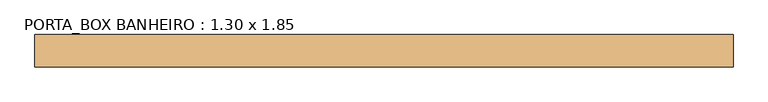
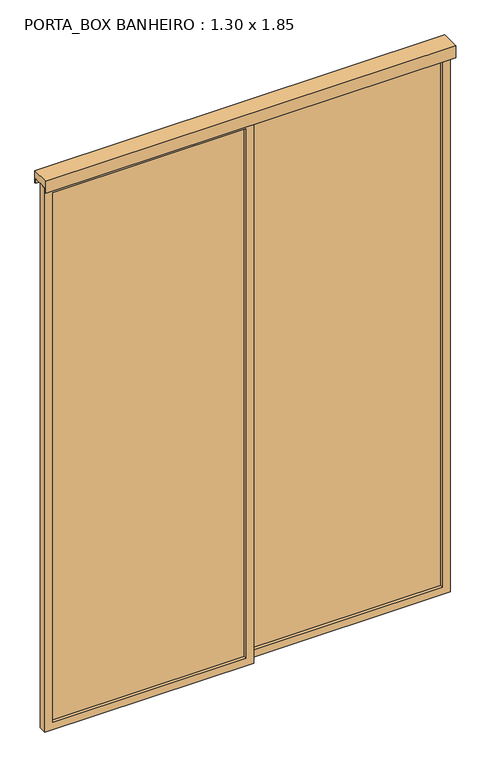
"""IFC4 building model written with IfcOpenShell, lengths in millimetres: door geometry, PORTA_BOX BANHEIRO : 1.30 x 1.85."""

from ifc_helpers import new_model, si_unit, frame, origin, place, context, project, spatial, polyline, outline, extrude, faceted_brep, source, transform, mapped, element, save


def porta_box_banheiro_1_30_x_1_85_4d29e14f(model_context):
    return source(origin(), model_context, "Body", "SolidModel", [
        extrude(outline(polyline([(652.5, 15.0), (652.5, 10.0), (10.0, 10.0), (10.0, 15.0), (652.5, 15.0)])), frame((0.0, 0.0, 10.0), z_axis=(0.0, 0.0, 1.0), x_axis=(1.0, 0.0, 0.0)), (0.0, 0.0, 1.0), 1805.0),
        faceted_brep([(637.5, 15.0, 1800.0), (637.5, 25.0, 1800.0), (637.5, 25.0, 25.0), (637.5, 15.0, 25.0), (662.5, 25.0, 1825.0), (662.5, 25.0, 0.0), (0.0, 25.0, 0.0), (0.0, 25.0, 1825.0), (25.0, 25.0, 1800.0), (25.0, 25.0, 25.0), (25.0, 15.0, 25.0), (10.0, 15.0, 1815.0), (10.0, 15.0, 10.0), (652.5, 15.0, 10.0), (652.5, 15.0, 1815.0), (25.0, 15.0, 1800.0), (662.5, 0.0, 1825.0), (662.5, 0.0, 0.0), (0.0, 0.0, 1825.0), (0.0, 0.0, 0.0), (637.5, 0.0, 1800.0), (637.5, 0.0, 25.0), (25.0, 0.0, 25.0), (25.0, 0.0, 1800.0), (637.5, 10.0, 1800.0), (637.5, 10.0, 25.0), (25.0, 10.0, 25.0), (25.0, 10.0, 1800.0), (652.5, 10.0, 1815.0), (652.5, 10.0, 10.0), (10.0, 10.0, 10.0), (10.0, 10.0, 1815.0)], [[[0, 1, 2, 3]], [[4, 5, 6, 7], [8, 9, 2, 1]], [[3, 2, 9, 10]], [[11, 12, 13, 14], [0, 3, 10, 15]], [[4, 16, 17, 5]], [[18, 19, 17, 16], [20, 21, 22, 23]], [[5, 17, 19, 6]], [[10, 9, 8, 15]], [[6, 19, 18, 7]], [[20, 24, 25, 21]], [[21, 25, 26, 22]], [[22, 26, 27, 23]], [[28, 14, 13, 29]], [[29, 13, 12, 30]], [[28, 29, 30, 31], [27, 26, 25, 24]], [[30, 12, 11, 31]], [[15, 8, 1, 0]], [[7, 18, 16, 4]], [[31, 11, 14, 28]], [[23, 27, 24, 20]]]),
        extrude(outline(polyline([(1290.0, 40.0), (1290.0, 35.0), (647.5, 35.0), (647.5, 40.0), (1290.0, 40.0)])), frame((0.0, 0.0, 10.0), z_axis=(0.0, 0.0, 1.0), x_axis=(1.0, 0.0, 0.0)), (0.0, 0.0, 1.0), 1805.0),
        faceted_brep([(1275.0, 40.0, 1800.0), (1275.0, 50.0, 1800.0), (1275.0, 50.0, 25.0), (1275.0, 40.0, 25.0), (1300.0, 50.0, 1825.0), (1300.0, 50.0, 0.0), (637.5, 50.0, 0.0), (637.5, 50.0, 1825.0), (662.5, 50.0, 1800.0), (662.5, 50.0, 25.0), (662.5, 40.0, 25.0), (647.5, 40.0, 1815.0), (647.5, 40.0, 10.0), (1290.0, 40.0, 10.0), (1290.0, 40.0, 1815.0), (662.5, 40.0, 1800.0), (1300.0, 25.0, 1825.0), (1300.0, 25.0, 0.0), (637.5, 25.0, 1825.0), (637.5, 25.0, 0.0), (1275.0, 25.0, 1800.0), (1275.0, 25.0, 25.0), (662.5, 25.0, 25.0), (662.5, 25.0, 1800.0), (1275.0, 35.0, 1800.0), (1275.0, 35.0, 25.0), (662.5, 35.0, 25.0), (662.5, 35.0, 1800.0), (1290.0, 35.0, 1815.0), (1290.0, 35.0, 10.0), (647.5, 35.0, 10.0), (647.5, 35.0, 1815.0)], [[[0, 1, 2, 3]], [[4, 5, 6, 7], [8, 9, 2, 1]], [[3, 2, 9, 10]], [[11, 12, 13, 14], [0, 3, 10, 15]], [[4, 16, 17, 5]], [[18, 19, 17, 16], [20, 21, 22, 23]], [[5, 17, 19, 6]], [[10, 9, 8, 15]], [[6, 19, 18, 7]], [[20, 24, 25, 21]], [[21, 25, 26, 22]], [[22, 26, 27, 23]], [[28, 14, 13, 29]], [[29, 13, 12, 30]], [[28, 29, 30, 31], [27, 26, 25, 24]], [[30, 12, 11, 31]], [[15, 8, 1, 0]], [[7, 18, 16, 4]], [[31, 11, 14, 28]], [[23, 27, 24, 20]]]),
        extrude(outline(polyline([(-5.0, 1810.0), (-5.0, 1850.0), (55.0, 1850.0), (55.0, 1810.0), (50.0, 1810.0), (50.0, 1825.0), (0.0, 1825.0), (0.0, 1810.0), (-5.0, 1810.0)])), frame((0.0, 0.0, 0.0), z_axis=(1.0, 0.0, 0.0), x_axis=(0.0, 1.0, 0.0)), (0.0, 0.0, 1.0), 1300.0),
    ])


if __name__ == "__main__":
    model = new_model("IFC4")
    model_context = context("Model", 3, world=origin())
    ifc_project = project(units=[si_unit("LENGTHUNIT", "METRE", prefix="MILLI")], contexts=[model_context])
    site = spatial("IfcSite", under=ifc_project)
    building = spatial("IfcBuilding", under=site)
    placement = place(None, origin())
    porta_box_banheiro_1_30_x_1_85_shape = porta_box_banheiro_1_30_x_1_85_4d29e14f(model_context)
    element("IfcDoor", 1, ObjectType="PORTA_BOX BANHEIRO : 1.30 x 1.85", at=placement, inside=building, context=model_context, shape_type="MappedRepresentation", body=[
        mapped(porta_box_banheiro_1_30_x_1_85_shape, transform((0.0, 0.0, 0.0), x_axis=(1.0, 0.0, 0.0), y_axis=(0.0, 1.0, 0.0), z_axis=(0.0, 0.0, 1.0))),
    ])
    save(model, "model.ifc")

# Revit data of these elements
# Type "PORTA_BOX BANHEIRO : 1.30 x 1.85"
#   Type Mark = "BOX"
#   Width = 1.30 m
#   Material montante = .ALUMÍNIO
#   Materia vidro = .VIDRO
# Element 1 (IfcDoor, "PORTA_BOX BANHEIRO : 1.30 x 1.85")
#   Materials on its faces: ".ALUMÍNIO", ".VIDRO"
# Materials
#   ".ALUMÍNIO": class "CC_METAIS", colour RGB 244 244 244, transparency 0, Description = "Material alumínio", Cost = 0
#   ".VIDRO": class "Genérico", colour RGB 198 236 255, transparency 0.95, Cost = 0
